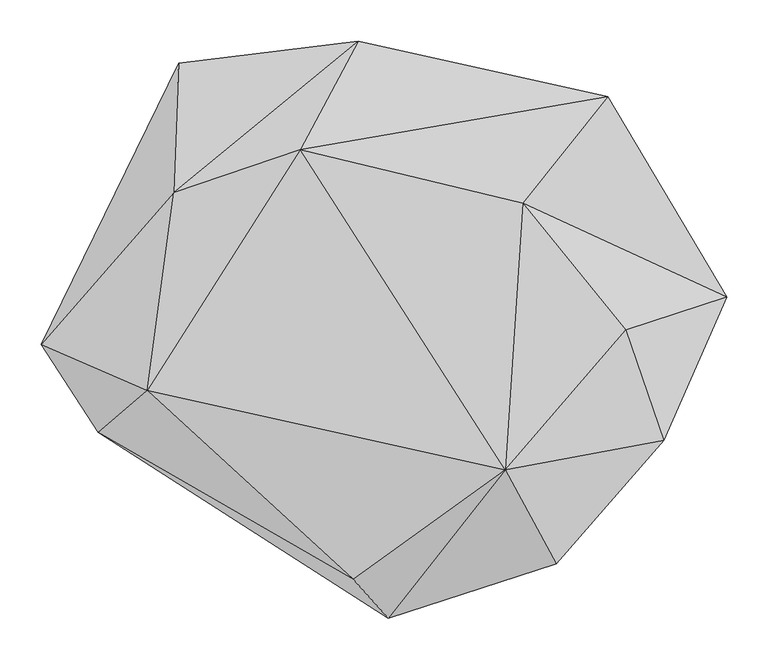
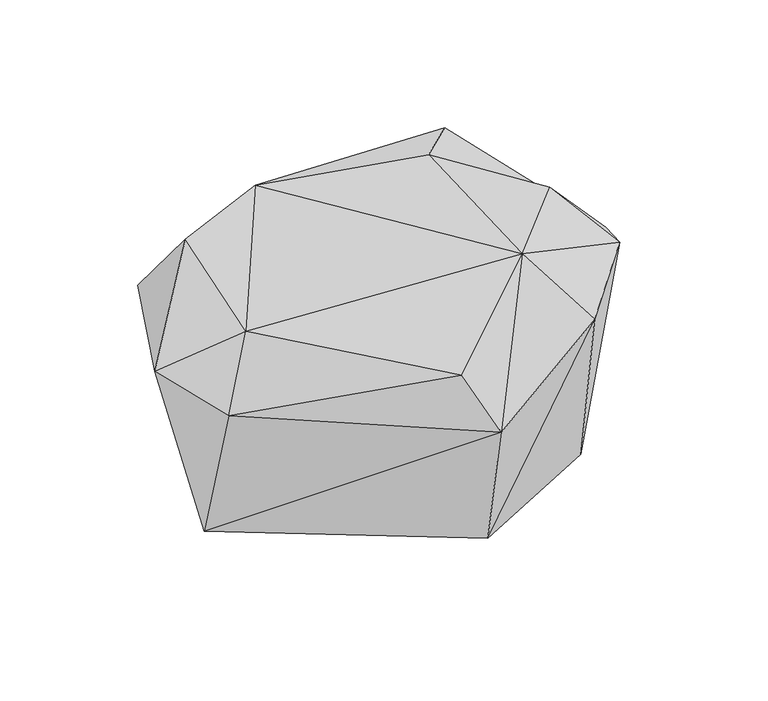
"""IFC4 building model written with IfcOpenShell, lengths in millimetres: geographic element geometry, Enscape AssetDefinition - Bush 072 Curry Plant : Enscape AssetDefinition - Bush 072 Curry Plant."""

from ifc_helpers import new_model, si_unit, origin, place, context, project, spatial, faceted_brep, source, transform, mapped, element, save


def geographic_element_405ae2fd(model_context):
    return source(origin(), model_context, "Body", "Brep", [
        faceted_brep([(-146.8649954, 238.4330034, 380.2570105), (-300.1939952, 186.3670051, 364.3870056), (-332.1230114, -53.6440015, 349.1620123), (-293.7940061, 343.3479965, 181.3939959), (-460.4279995, 2.2829999, 285.2959931), (-76.4309987, 369.6419895, 253.5279989), (122.4860027, 173.1619984, 382.6189935), (225.5720049, 302.7560115, 317.7419901), (101.365, -149.9080062, 400.4740119), (-69.953002, 328.1089962, 0.0), (195.182994, 269.3879902, 0.0), (-281.8869948, 277.9330015, 0.0), (-255.1580071, 92.7840024, -63.4969994), (-16.2450001, 57.0480004, -63.4969994), (321.8550086, 55.7609983, 0.0), (197.5920051, -162.4550074, 0.0), (-38.1140001, -285.9129906, 0.0), (-404.2370021, -51.9299991, 0.0), (-391.5250003, -104.6250015, 243.3490008), (-40.1649997, -329.7609985, 225.6450057), (163.240999, -263.7999952, 325.5439997), (-82.6319978, -282.656014, 318.5259998), (293.3920026, -114.4710034, 333.0079913), (247.2939938, 19.8219996, 370.4890013), (369.8579967, 59.4240017, 229.4670045)], [[[0, 1, 2]], [[1, 3, 4]], [[1, 4, 2]], [[0, 5, 1]], [[1, 5, 3]], [[6, 7, 0]], [[0, 8, 6]], [[0, 2, 8]], [[0, 7, 5]], [[9, 5, 10]], [[9, 3, 5]], [[10, 5, 7]], [[11, 3, 9]], [[11, 4, 3]], [[12, 11, 9]], [[13, 9, 10]], [[12, 9, 13]], [[10, 7, 14]], [[13, 10, 14]], [[13, 14, 15]], [[13, 15, 16]], [[13, 16, 12]], [[12, 17, 11]], [[12, 16, 17]], [[17, 4, 11]], [[17, 18, 4]], [[16, 19, 17]], [[17, 19, 18]], [[15, 20, 16]], [[16, 20, 19]], [[21, 19, 8]], [[21, 18, 19]], [[8, 19, 20]], [[2, 18, 21]], [[2, 4, 18]], [[8, 2, 21]], [[8, 20, 22]], [[8, 22, 23]], [[6, 8, 23]], [[15, 22, 20]], [[23, 22, 24]], [[15, 24, 22]], [[23, 24, 6]], [[6, 24, 7]], [[14, 24, 15]], [[14, 7, 24]]]),
    ])


if __name__ == "__main__":
    model = new_model("IFC4")
    model_context = context("Model", 3, world=origin())
    ifc_project = project(units=[si_unit("LENGTHUNIT", "METRE", prefix="MILLI")], contexts=[model_context])
    site = spatial("IfcSite", under=ifc_project)
    building = spatial("IfcBuilding", under=site)
    placement = place(None, origin())
    geographic_element_shape = geographic_element_405ae2fd(model_context)
    element("IfcGeographicElement", 1, ObjectType="Enscape AssetDefinition - Bush 072 Curry Plant : Enscape AssetDefinition - Bush 072 Curry Plant", at=placement, inside=building, context=model_context, shape_type="MappedRepresentation", body=[
        mapped(geographic_element_shape, transform((0.0, 0.0, 0.0), x_axis=(1.0, 0.0, 0.0), y_axis=(0.0, 1.0, 0.0), z_axis=(0.0, 0.0, 1.0))),
    ])
    save(model, "model.ifc")

# Revit data of these elements
# Type "Enscape AssetDefinition - Bush 072 Curry Plant : Enscape AssetDefinition - Bush 072 Curry Plant"
#   EnscapeAssetSource = "REMOTE"
#   EnscapeAssetId = "15e17545-df46-4152-8e9d-9cf5b3541e6d"
#   Height = 0.400474 m
#   EnscapeNativeAssetHeight = 0.400474 m
#   Default Elevation = 0
